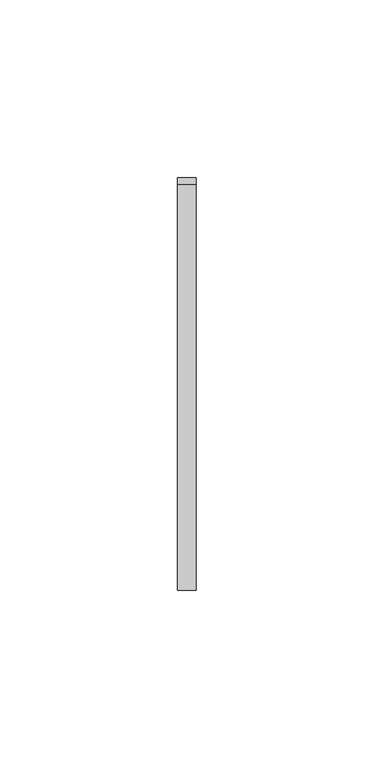
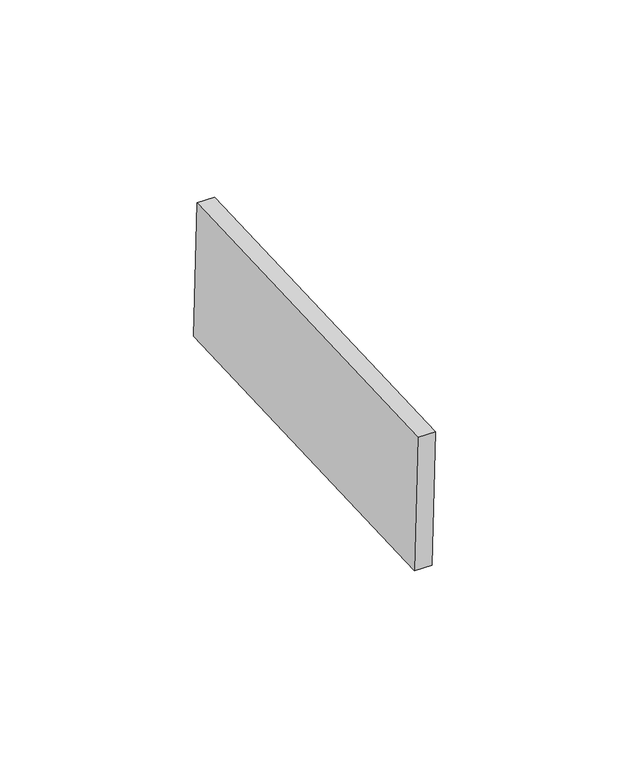
"""IFC4 building model written with IfcOpenShell, lengths in millimetres: proxy geometry, Inner panel:Inner panel:1:Inner panel:1 : Inner panel:Inner panel:300324:2:Inner panel:1:Inner panel:1 : Inner panel:Inner panel:300324:2 : Inner panel:Inner panel:1:Inner panel:1 : Inner panel:Inner panel:300324:300043:54 : Inner panel:Inner panel:1:Inner panel:1 : Inner panel:Inner panel:300324:2:Inner panel:1:Inner panel:1 : Inner panel:Inner panel:300324:2 : Inner panel:Inner panel:1:Inner panel:1 : Inner panel:Inner panel:300324:300043:308120."""

from ifc_helpers import new_model, si_unit, frame, origin, place, context, project, spatial, polyline, outline, extrude, source, transform, mapped, element, save


def generic_models_f6d3cb04(model_context):
    return source(origin(), model_context, "Body", "SweptSolid", [
        extrude(outline(polyline([(0.0, -114.2999999), (0.0, 0.0), (5.2138089, 0.0), (5.2138089, -114.2999999), (0.0, -114.2999999)])), frame((592310.995117, -566950.1308393, 8857.6957503), z_axis=(0.0, -0.04163054471215927, 0.9991330730923529), x_axis=(-1.0, 0.0, 0.0)), (0.0, 0.0, 1.0), 43.2233908),
    ])


if __name__ == "__main__":
    model = new_model("IFC4")
    model_context = context("Model", 3, world=origin())
    ifc_project = project(units=[si_unit("LENGTHUNIT", "METRE", prefix="MILLI")], contexts=[model_context])
    site = spatial("IfcSite", under=ifc_project)
    building = spatial("IfcBuilding", under=site)
    placement = place(None, origin())
    generic_models_shape = generic_models_f6d3cb04(model_context)
    element("IfcBuildingElementProxy", 1, Name="Inner panel:Inner panel:1:Inner panel:1 : Inner panel:Inner panel:300324:2:Inner panel:1:Inner panel:1 : Inner panel:Inner panel:300324:2 : Inner panel:Inner panel:1:Inner panel:1 : Inner panel:Inner panel:300324:300043:54 : Inner panel:Inner panel:1:Inner panel:1 : Inner panel:Inner panel:300324:2:Inner panel:1:Inner panel:1 : Inner panel:Inner panel:300324:2 : Inner panel:Inner panel:1:Inner panel:1 : Inner panel:Inner panel:300324:300043:308120", ObjectType="Inner panel:Inner panel:1:Inner panel:1 : Inner panel:Inner panel:300324:2:Inner panel:1:Inner panel:1 : Inner panel:Inner panel:300324:2 : Inner panel:Inner panel:1:Inner panel:1 : Inner panel:Inner panel:300324:300043:54 : Inner panel:Inner panel:1:Inner panel:1 : Inner panel:Inner panel:300324:2:Inner panel:1:Inner panel:1 : Inner panel:Inner panel:300324:2 : Inner panel:Inner panel:1:Inner panel:1 : Inner panel:Inner panel:300324:300043:308120", at=placement, inside=building, context=model_context, shape_type="MappedRepresentation", body=[
        mapped(generic_models_shape, transform((0.0, 0.0, 0.0), x_axis=(1.0, 0.0, 0.0), y_axis=(0.0, 1.0, 0.0), z_axis=(0.0, 0.0, 1.0))),
    ])
    save(model, "model.ifc")

# Revit data of these elements
# Type "Inner panel:Inner panel:1:Inner panel:1 : Inner panel:Inner panel:300324:2:Inner panel:1:Inner panel:1 : Inner panel:Inner panel:300324:2 : Inner panel:Inner panel:1:Inner panel:1 : Inner panel:Inner panel:300324:300043:54 : Inner panel:Inner panel:1:Inner panel:1 : Inner panel:Inner panel:300324:2:Inner panel:1:Inner panel:1 : Inner panel:Inner panel:300324:2 : Inner panel:Inner panel:1:Inner panel:1 : Inner panel:Inner panel:300324:300043:308120"
#   NameOverride = "Inner panel:Inner panel:1:Inner panel:1 : Inner panel:Inner panel:300324:2:Inner panel:1:Inner panel:1 : Inner panel:Inner panel:300324:2 : Inner panel:Inner panel:1:Inner panel:1 : Inner panel:Inner panel:300324:300043:308120"
#   ObjectTypeOverride = "Inner panel:1:Inner panel:1 : Inner panel:Inner panel:300324:2 : Inner panel:Inner panel:1:Inner panel:1 : Inner panel:Inner panel:300324:300043"
#   Reference = "Inner panel"
#   Tag = "308120"
# Element 1 (IfcBuildingElementProxy, "Inner panel:Inner panel:1:Inner panel:1 : Inner panel:Inner panel:300324:2:Inner panel:1:Inner panel:1 : Inner panel:Inner panel:300324:2 : Inner panel:Inner panel:1:Inner panel:1 : Inner panel:Inner panel:300324:300043:54 : Inner panel:Inner panel:1:Inner panel:1 : Inner panel:Inner panel:300324:2:Inner panel:1:Inner panel:1 : Inner panel:Inner panel:300324:2 : Inner panel:Inner panel:1:Inner panel:1 : Inner panel:Inner panel:300324:300043:308120")
#   Materials on its faces: "SLIDING CLIP"
# Materials
#   "SLIDING CLIP": class "Generic", colour RGB 120 120 120, transparency 0, Cost = 0
